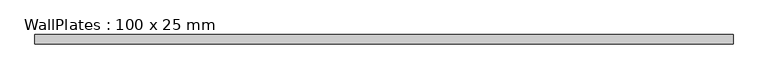
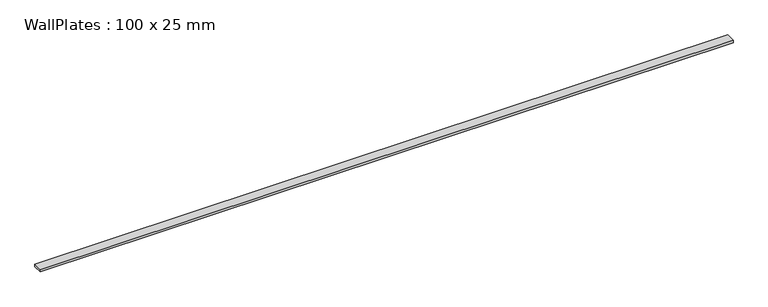
"""IFC4 building model written with IfcOpenShell, lengths in millimetres: beam geometry, WallPlates : 100 x 25 mm."""

from ifc_helpers import new_model, si_unit, frame, origin, place, context, project, spatial, polyline, outline, extrude, source, transform, mapped, element, save


def wallplates_100_x_25_mm_b6c8317b(model_context):
    return source(origin(), model_context, "Body", "SweptSolid", [
        extrude(outline(polyline([(-3600.0, -50.0), (-3600.0, 50.0), (3700.0, 50.0), (3700.0, -50.0), (-3600.0, -50.0)])), frame((0.0, 0.0, -12.5), z_axis=(0.0, 0.0, 1.0), x_axis=(1.0, 0.0, 0.0)), (0.0, 0.0, 1.0), 25.0),
    ])


if __name__ == "__main__":
    model = new_model("IFC4")
    model_context = context("Model", 3, world=origin())
    ifc_project = project(units=[si_unit("LENGTHUNIT", "METRE", prefix="MILLI")], contexts=[model_context])
    site = spatial("IfcSite", under=ifc_project)
    building = spatial("IfcBuilding", under=site)
    placement = place(None, origin())
    wallplates_100_x_25_mm_shape = wallplates_100_x_25_mm_b6c8317b(model_context)
    element("IfcBeam", 1, ObjectType="WallPlates : 100 x 25 mm", at=placement, inside=building, context=model_context, shape_type="MappedRepresentation", body=[
        mapped(wallplates_100_x_25_mm_shape, transform((0.0, 0.0, 0.0), x_axis=(1.0, 0.0, 0.0), y_axis=(0.0, 1.0, 0.0), z_axis=(0.0, 0.0, 1.0))),
    ])
    save(model, "model.ifc")

# Revit data of these elements
# Type "WallPlates : 100 x 25 mm"
#   ExpertTruss = "Height\th\r\nWidth\tb"
#   Name [instance default] = ""
#   m [instance default] = 0 mm
#   ip_c_cut [instance default] = 1025 mm
#   h_fix [instance default] = 75 mm
#   d/2 [instance default] = 1750 mm
#   c_cut_incl [instance default] = -1000 mm
#   c_cut [instance default] = 0 mm
#   alfaMax [instance default] = 0.00°
#   alfa0_2 [instance default] = 90.00°
#   Alfa_str [instance default] = 0.00°
#   Alfa_cut [instance default] = 90.00°
#   AlfaMAX [instance default] = 0.00°
#   Alfa2_0 [instance default] = 0.00°
#   Alfa2 [instance default] = 0.00°
#   Alfa1_0 [instance default] = 0.00°
#   Alfa1 [instance default] = 0.00°
#   A_max_Str [instance default] = 0.00°
#   h_void [instance default] = 25 mm
#   beam_L_0 [instance default] = 100 mm
#   beam_L [instance default] = 0 mm
#   b_void [instance default] = 110 mm
#   alfa0_1 [instance default] = 90.00°
#   b = 100 mm
#   YOffsetStr [instance default] = 0 mm
#   YOffsetEnd [instance default] = 0 mm
#   XOffsetStr_0 [instance default] = 3500 mm
#   XOffsetStr [instance default] = 0 mm
#   XOffsetEnd_0 [instance default] = 3500 mm
#   XOffsetEnd [instance default] = 0 mm
#   L_void_0 [instance default] = 100 mm
#   L_void [instance default] = 0 mm
#   E2 [instance default] = 0.00°
#   E1 [instance default] = 0.00°
#   Length [instance default] = 3500 mm
#   h = 25 mm
#   Alfa [instance default] = 0.00°
#   A_max_End [instance default] = 0.00°
#   A_max [instance default] = 0.00°
#   A4 [instance default] = 0.00°
#   A3 [instance default] = 0.00°
#   A2 [instance default] = 0.00°
#   A1 [instance default] = 0.00°
#   Material [instance default] = Wood Standard
# Element 1 (IfcBeam, "WallPlates : 100 x 25 mm")
#   d/2 = 3650 mm
#   XOffsetStr_0 = 7250 mm
#   XOffsetStr = 50 mm
#   XOffsetEnd_0 = 7350 mm
#   XOffsetEnd = -50 mm
#   Materials on its faces: "Wood Standard"
# Materials
#   "Wood Standard": class "Drewno", colour RGB 196 146 67, transparency 0, Cost = 0
